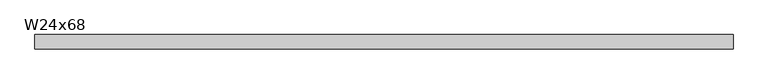
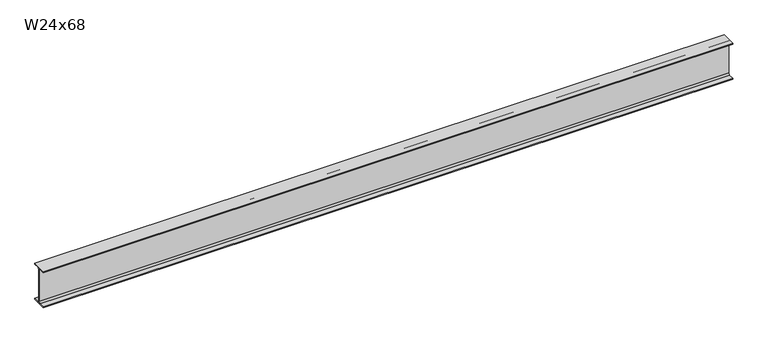
"""IFC4 building model written with IfcOpenShell, lengths in millimetres: beam geometry, RME W-Wide Flange : W24x68."""

from ifc_helpers import new_model, si_unit, point, frame, frame_2d, origin, place, context, project, spatial, polyline, circle_curve, trimmed, segment, composite_curve, outline, extrude, source, transform, mapped, element, save


def w24x68_5022dcac(model_context):
    return source(origin(), model_context, "Body", "SweptSolid", [
        extrude(outline(composite_curve([segment(polyline([(113.919, -286.131), (113.919, -300.99), (-113.919, -300.99), (-113.919, -286.131), (-28.5115, -286.131)]), True, "CONTINUOUS"), segment(trimmed(circle_curve(frame_2d((-28.5115, -262.89)), 23.241), [point((-28.5115, -286.131))], [point((-5.2705, -262.89))], True, "CARTESIAN"), True, "CONTINUOUS"), segment(polyline([(-5.2705, -262.89), (-5.2705, 262.89)]), True, "CONTINUOUS"), segment(trimmed(circle_curve(frame_2d((-28.5115, 262.89)), 23.241), [point((-5.2705, 262.89))], [point((-28.5115, 286.131))], True, "CARTESIAN"), True, "CONTINUOUS"), segment(polyline([(-28.5115, 286.131), (-113.919, 286.131), (-113.919, 300.99), (113.919, 300.99), (113.919, 286.131), (28.5115, 286.131)]), True, "CONTINUOUS"), segment(trimmed(circle_curve(frame_2d((28.5115, 262.89)), 23.241), [point((28.5115, 286.131))], [point((5.2705, 262.89))], True, "CARTESIAN"), True, "CONTINUOUS"), segment(polyline([(5.2705, 262.89), (5.2705, -262.89)]), True, "CONTINUOUS"), segment(trimmed(circle_curve(frame_2d((28.5115, -262.89)), 23.241), [point((5.2705, -262.89))], [point((28.5115, -286.131))], True, "CARTESIAN"), True, "CONTINUOUS"), segment(polyline([(28.5115, -286.131), (113.919, -286.131)]), True, "CONTINUOUS")], self_intersect=False)), frame((-5440.5550445, 0.0, 0.0), z_axis=(1.0, 0.0, 0.0), x_axis=(0.0, 1.0, 0.0)), (0.0, 0.0, 1.0), 10916.4922976),
    ])


if __name__ == "__main__":
    model = new_model("IFC4")
    model_context = context("Model", 3, world=origin())
    ifc_project = project(units=[si_unit("LENGTHUNIT", "METRE", prefix="MILLI")], contexts=[model_context])
    site = spatial("IfcSite", under=ifc_project)
    building = spatial("IfcBuilding", under=site)
    placement = place(None, origin())
    w24x68_shape = w24x68_5022dcac(model_context)
    element("IfcBeam", 1, ObjectType="RME W-Wide Flange : W24x68", at=placement, inside=building, context=model_context, shape_type="MappedRepresentation", body=[
        mapped(w24x68_shape, transform((0.0, 0.0, 0.0), x_axis=(1.0, 0.0, 0.0), y_axis=(0.0, 1.0, 0.0), z_axis=(0.0, 0.0, 1.0))),
    ])
    save(model, "model.ifc")

# Revit data of these elements
# Type "RME W-Wide Flange : W24x68"
#   WELD P [instance default] = ""
#   WELD LE [instance default] = ""
#   WELD D [instance default] = ""
#   TOP SECTION SIZE [instance default] = ""
#   TOP SECTION LENGTH [instance default] = ""
#   REMARKS [instance default] = ""
#   REINF TYPE [instance default] = ""
#   Nominal Size = "W24"
#   End Bearing Capacity [instance default] = ""
#   BOT SECTION SIZE [instance default] = ""
#   BOT SECTION LENGTH [instance default] = ""
#   Assembly Code = "B10"
#   W = 68
#   Start Extension Calculation [instance default] = 10' - 0"
#   Start Extension [instance default] = -0' - 0 1/2"
#   End Extension Calculation [instance default] = 10' - 0"
#   End Extension [instance default] = -0' - 0 1/2"
#   Length [instance default] = 5' - 0"
#   bf = 0' - 8.97"
#   d = 1' - 11.7"
#   k = 0' - 1 1/2"
#   k2 = 0' - 0.915"
#   tf = 0' - 0.585"
#   tw = 0' - 0.415"
#   A = 0.139583 SF
#   Structural Material [instance default] = Metal - Steel - ASTM A992
# Element 1 (IfcBeam, "RME W-Wide Flange : W24x68")
#   Length = 36' - 0.17616"
#   Materials on its faces: "Metal - Steel - ASTM A992"
# Materials
#   "Metal - Steel - ASTM A992": class "Metal", colour RGB 255 128 0, transparency 0
